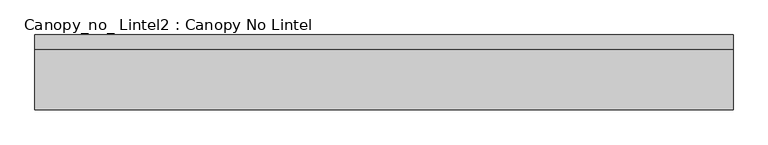
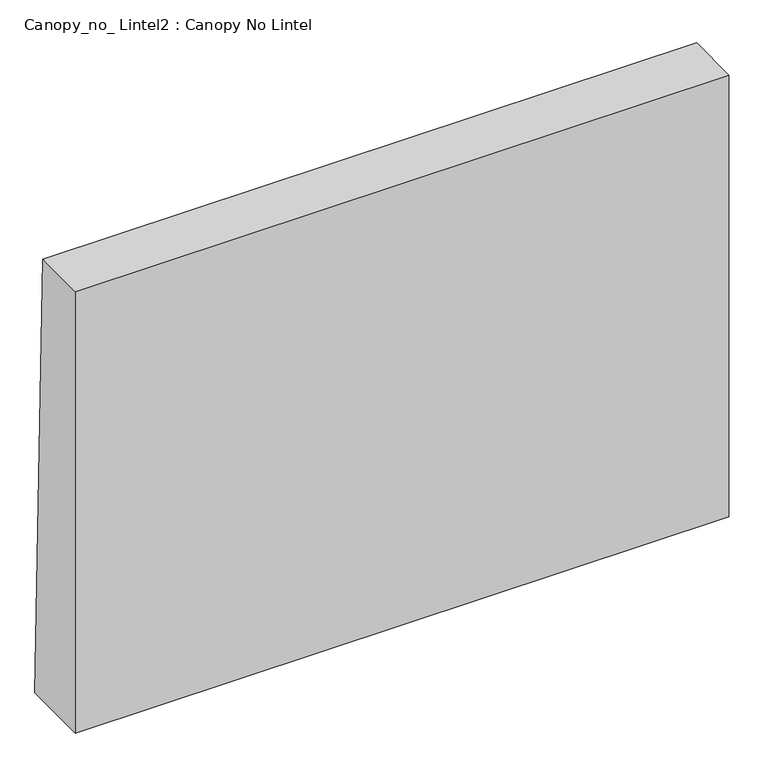
"""IFC4 building model written with IfcOpenShell, lengths in millimetres: proxy geometry, Canopy_no_ Lintel2 : Canopy No Lintel."""

from ifc_helpers import new_model, si_unit, frame, origin, place, context, project, spatial, polyline, outline, extrude, source, transform, mapped, element, save


def canopy_no_lintel2_canopy_no_lintel_90d8ac49(model_context):
    return source(origin(), model_context, "Body", "SweptSolid", [
        extrude(outline(polyline([(-30.0, 1000.0), (0.0, 0.0), (-150.0, 0.0), (-150.0, 1000.0), (-30.0, 1000.0)])), frame((0.0, 0.0, 0.0), z_axis=(1.0, 0.0, 0.0), x_axis=(0.0, 1.0, 0.0)), (0.0, 0.0, 1.0), 1400.0),
    ])


if __name__ == "__main__":
    model = new_model("IFC4")
    model_context = context("Model", 3, world=origin())
    ifc_project = project(units=[si_unit("LENGTHUNIT", "METRE", prefix="MILLI")], contexts=[model_context])
    site = spatial("IfcSite", under=ifc_project)
    building = spatial("IfcBuilding", under=site)
    placement = place(None, origin())
    canopy_no_lintel2_canopy_no_lintel_shape = canopy_no_lintel2_canopy_no_lintel_90d8ac49(model_context)
    element("IfcBuildingElementProxy", 1, Name="Canopy_no_ Lintel2 : Canopy No Lintel", ObjectType="Canopy_no_ Lintel2 : Canopy No Lintel", at=placement, inside=building, context=model_context, shape_type="MappedRepresentation", body=[
        mapped(canopy_no_lintel2_canopy_no_lintel_shape, transform((0.0, 0.0, 0.0), x_axis=(1.0, 0.0, 0.0), y_axis=(0.0, 1.0, 0.0), z_axis=(0.0, 0.0, 1.0))),
    ])
    save(model, "model.ifc")

# Revit data of these elements
# Type "Canopy_no_ Lintel2 : Canopy No Lintel"
#   LastUpdate = "2017-07-05 오후 5:00:05"
#   EditorName = ""
#   lintel width = 413 mm
#   lintel edge = 0 mm
#   lintel depth = 400 mm
#   d2 = 150 mm
#   d1 = 30 mm
#   W = 1000 mm
#   Length [instance default] = 2000 mm
#   Default Elevation = 1219.2 mm
#   Structure Material = none
# Element 1 (IfcBuildingElementProxy, "Canopy_no_ Lintel2 : Canopy No Lintel")
#   Length = 1400 mm
